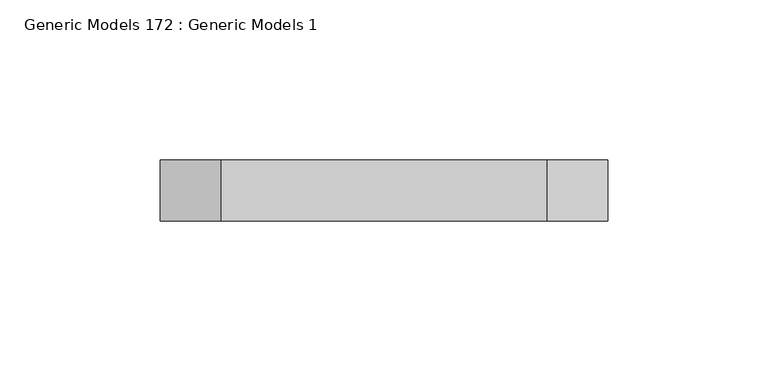
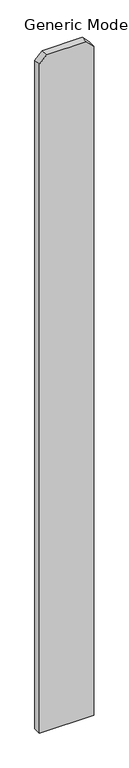
"""IFC4 building model written with IfcOpenShell, lengths in millimetres: proxy geometry, Generic Models 172 : Generic Models 1."""

import ifcopenshell
import ifcopenshell.guid

model = None  # the IFC model being written
_history = None  # IfcOwnerHistory: only IFC2X3 demands one
_inside = {}  # id of a spatial element -> (the spatial element, [elements in it])
_under = {}  # id of a project, library or spatial element -> (it, [spatial elements below it])
_declared = {}  # id of a project -> (the project, [libraries it declares])
_typed = {}  # id of a type object -> (the type object, [elements of that type])
_made_of = {}  # id of a material, layer set ... -> (it, [elements and type objects made of it])


def new_model(schema):
    """Start an empty IFC model of exactly this schema.

    Asked for "IFC4X3", IfcOpenShell would pick the latest addendum, in which some entities
    have other attributes; the version numbers below select the first issue.
    IFC2X3 requires an IfcOwnerHistory on every rooted entity: one is made here for all.
    """
    global model, _history
    if schema == "IFC4X3":
        model = ifcopenshell.file(schema_version=(4, 3, 0, 0))
    else:
        model = ifcopenshell.file(schema=schema)
    _inside.clear()
    _under.clear()
    _declared.clear()
    _typed.clear()
    _made_of.clear()
    _history = None
    if model.schema == "IFC2X3":
        org = make("IfcOrganization", Name="unknown")
        user = make(
            "IfcPersonAndOrganization",
            ThePerson=make("IfcPerson", FamilyName="unknown"),
            TheOrganization=org,
        )
        app = make(
            "IfcApplication",
            ApplicationDeveloper=org,
            Version="unknown",
            ApplicationFullName="unknown",
            ApplicationIdentifier="unknown",
        )
        _history = make(
            "IfcOwnerHistory",
            OwningUser=user,
            OwningApplication=app,
            ChangeAction="ADDED",
            CreationDate=0,
        )
    return model


def make(cls, **values):
    """One entity of the class cls with the attributes given. An attribute that is None is left unset."""
    return model.create_entity(
        cls, **{name: value for name, value in values.items() if value is not None}
    )


def rooted(cls, **values):
    """An entity with a GlobalId (a new one), such as an element, a storey or a relation."""
    return make(cls, GlobalId=ifcopenshell.guid.new(), OwnerHistory=_history, **values)


def si_unit(unit_type, name, prefix=None):
    """IfcSIUnit, for example si_unit("LENGTHUNIT", "METRE", prefix="MILLI")."""
    return make("IfcSIUnit", UnitType=unit_type, Prefix=prefix, Name=name)


def assignment(units):
    """IfcUnitAssignment: the units of a project."""
    return None if units is None else make("IfcUnitAssignment", Units=units)


def point(xyz):
    """IfcCartesianPoint."""
    return None if xyz is None else make("IfcCartesianPoint", Coordinates=xyz)


def direction(xyz):
    """IfcDirection."""
    return None if xyz is None else make("IfcDirection", DirectionRatios=xyz)


def frame(location, z_axis=None, x_axis=None):
    """IfcAxis2Placement3D, a coordinate frame: its origin and axes. An axis left out is left unset."""
    return make(
        "IfcAxis2Placement3D",
        Location=point(location),
        Axis=direction(z_axis),
        RefDirection=direction(x_axis),
    )


def origin():
    """The frame at (0, 0, 0) with its axes left unset."""
    return frame((0.0, 0.0, 0.0))


def place(relative_to, where):
    """IfcLocalPlacement: puts the frame where relative to a parent placement (None: the world)."""
    return make(
        "IfcLocalPlacement", PlacementRelTo=relative_to, RelativePlacement=where
    )


def context(
    kind, dimensions, precision=None, world=None, true_north=None, identifier=None
):
    """IfcGeometricRepresentationContext, for example the 3D "Model" context."""
    return make(
        "IfcGeometricRepresentationContext",
        ContextIdentifier=identifier,
        ContextType=kind,
        CoordinateSpaceDimension=dimensions,
        Precision=precision,
        WorldCoordinateSystem=world,
        TrueNorth=true_north,
    )


def project(units=None, contexts=None):
    """IfcProject with its units and contexts."""
    return rooted(
        "IfcProject",
        Name="project",
        RepresentationContexts=contexts,
        UnitsInContext=assignment(units),
    )


def spatial(cls, under=None, at=None, **own):
    """A site, building, storey or space (cls), placed at a placement, below another one or the project."""
    s = rooted(cls, ObjectPlacement=at, **own)
    if under is not None:
        _under.setdefault(under.id(), (under, []))[1].append(s)
    return s


def polyline(points):
    """IfcPolyline through the points."""
    return make("IfcPolyline", Points=[point(p) for p in points])


def outline(outer, holes=None, kind="AREA"):
    """IfcArbitraryClosedProfileDef: a profile drawn as a closed curve; with holes, ...WithVoids."""
    if holes is None:
        return make("IfcArbitraryClosedProfileDef", ProfileType=kind, OuterCurve=outer)
    return make(
        "IfcArbitraryProfileDefWithVoids",
        ProfileType=kind,
        OuterCurve=outer,
        InnerCurves=holes,
    )


def extrude(swept, where, along, depth):
    """IfcExtrudedAreaSolid: the profile swept, set in the frame where, extruded along a direction by depth."""
    return make(
        "IfcExtrudedAreaSolid",
        SweptArea=swept,
        Position=where,
        ExtrudedDirection=direction(along),
        Depth=depth,
    )


def shape(context_of_items, identifier, shape_type, items):
    """IfcShapeRepresentation: the items that make up one representation, for example the "Body"."""
    return make(
        "IfcShapeRepresentation",
        ContextOfItems=context_of_items,
        RepresentationIdentifier=identifier,
        RepresentationType=shape_type,
        Items=items,
    )


def source(mapping_origin, context_of_items, identifier, shape_type, items):
    """IfcRepresentationMap: a shape defined once, which mapped items show again and again."""
    return make(
        "IfcRepresentationMap",
        MappingOrigin=mapping_origin,
        MappedRepresentation=shape(context_of_items, identifier, shape_type, items),
    )


def transform(
    local_origin,
    x_axis=None,
    y_axis=None,
    z_axis=None,
    scale=None,
    scale2=None,
    scale3=None,
    uniform=True,
):
    """IfcCartesianTransformationOperator3D, or its non-uniform kind. x_axis, y_axis, z_axis: its Axis1, 2, 3."""
    if uniform:
        return make(
            "IfcCartesianTransformationOperator3D",
            Axis1=direction(x_axis),
            Axis2=direction(y_axis),
            LocalOrigin=point(local_origin),
            Scale=scale,
            Axis3=direction(z_axis),
        )
    return make(
        "IfcCartesianTransformationOperator3DnonUniform",
        Axis1=direction(x_axis),
        Axis2=direction(y_axis),
        LocalOrigin=point(local_origin),
        Scale=scale,
        Axis3=direction(z_axis),
        Scale2=scale2,
        Scale3=scale3,
    )


def mapped(mapping_source, mapping_target):
    """IfcMappedItem: shows the shape of a source again, moved by a transform."""
    return make(
        "IfcMappedItem", MappingSource=mapping_source, MappingTarget=mapping_target
    )


def made_of(thing, what):
    """Note that an element or type object is made of a material, layer set ...; save() writes the relation."""
    if what is not None:
        _made_of.setdefault(what.id(), (what, []))[1].append(thing)
    return thing


def element(
    cls,
    number,
    at=None,
    inside=None,
    cuts=None,
    type_object=None,
    material=None,
    context=None,
    identifier="Body",
    shape_type=None,
    held_by="IfcProductDefinitionShape",
    body=None,
    shapes=None,
    **own,
):
    """One element of the class cls, such as IfcWall. Its Tag is "e" and its number.

    at: its placement. inside: the storey or other place that contains it. cuts: it is an
    opening in that element (IfcRelVoidsElement). A single representation is given by context,
    identifier, shape_type and body (its items); several are given by shapes. held_by: the class
    of the entity that holds the representations. save() writes the other relations.
    """
    e = rooted(cls, Tag="e%d" % number, ObjectPlacement=at, **own)
    if body is not None:
        shapes = [shape(context, identifier, shape_type, body)]
    if shapes is not None:
        e.Representation = make(held_by, Representations=shapes)
    if inside is not None:
        _inside.setdefault(inside.id(), (inside, []))[1].append(e)
    if cuts is not None:
        rooted(
            "IfcRelVoidsElement", RelatingBuildingElement=cuts, RelatedOpeningElement=e
        )
    if type_object is not None:
        _typed.setdefault(type_object.id(), (type_object, []))[1].append(e)
    return made_of(e, material)


def aggregate(whole, parts):
    """IfcRelAggregates: a whole, such as a stair, and the parts it consists of."""
    return rooted("IfcRelAggregates", RelatingObject=whole, RelatedObjects=parts)


def save(model, path):
    """Write the relations noted so far, then the file.

    IfcRelAggregates (storeys below a building ...), IfcRelContainedInSpatialStructure (elements
    in a storey), IfcRelDefinesByType, IfcRelAssociatesMaterial and IfcRelDeclares: one each for
    every whole, place, type object, material and project.
    """
    for whole, parts in _under.values():
        aggregate(whole, parts)
    for where, things in _inside.values():
        rooted(
            "IfcRelContainedInSpatialStructure",
            RelatedElements=things,
            RelatingStructure=where,
        )
    for kind, things in _typed.values():
        rooted("IfcRelDefinesByType", RelatedObjects=things, RelatingType=kind)
    for what, things in _made_of.values():
        rooted("IfcRelAssociatesMaterial", RelatedObjects=things, RelatingMaterial=what)
    for by, libraries in _declared.values():
        rooted("IfcRelDeclares", RelatingContext=by, RelatedDefinitions=libraries)
    model.write(path)


def generic_models_172_generic_models_1_01be16c1(model_context):
    return source(origin(), model_context, "Body", "SweptSolid", [
        extrude(outline(polyline([(76.2, 56208.6125), (1885.95, 56208.6125), (1905.0, 56189.5625), (1905.0, 56087.9625), (1885.95, 56068.9125), (76.2, 56068.9125), (76.2, 56208.6125)])), frame((0.0, 547.6875, 0.0), z_axis=(0.0, 1.0, 0.0), x_axis=(0.0, 0.0, 1.0)), (0.0, 0.0, 1.0), 19.05),
    ])


if __name__ == "__main__":
    model = new_model("IFC4")
    model_context = context("Model", 3, world=origin())
    ifc_project = project(units=[si_unit("LENGTHUNIT", "METRE", prefix="MILLI")], contexts=[model_context])
    site = spatial("IfcSite", under=ifc_project)
    building = spatial("IfcBuilding", under=site)
    placement = place(None, origin())
    generic_models_172_generic_models_1_shape = generic_models_172_generic_models_1_01be16c1(model_context)
    element("IfcBuildingElementProxy", 1, Name="Generic Models 172 : Generic Models 1", ObjectType="Generic Models 172 : Generic Models 1", at=placement, inside=building, context=model_context, shape_type="MappedRepresentation", body=[
        mapped(generic_models_172_generic_models_1_shape, transform((0.0, 0.0, 0.0), x_axis=(1.0, 0.0, 0.0), y_axis=(0.0, 1.0, 0.0), z_axis=(0.0, 0.0, 1.0))),
    ])
    save(model, "model.ifc")

# Revit data of these elements
# Element 1 (IfcBuildingElementProxy, "Generic Models 172 : Generic Models 1")
#   Materials on its faces: "VERTICAL 1X6 CEDAR PLANKS W/ CLEAR WOOD SEALER"
# Materials
#   "VERTICAL 1X6 CEDAR PLANKS W/ CLEAR WOOD SEALER": class "Wood", colour RGB 234 198 147, transparency 0, Description = "Pinus Echinata", Cost = 0
